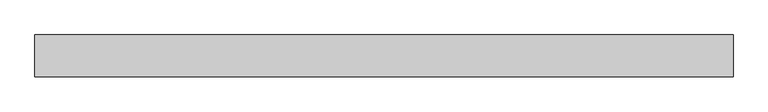
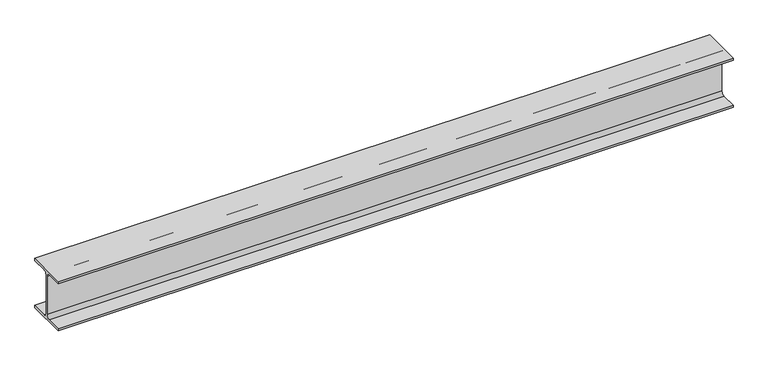
"""IFC4 building model written with IfcOpenShell, lengths in millimetres: beam geometry, 0912_Steel Framing_H-KSD3502 : H_SB_ASB_H-194x150x6x9."""

from ifc_helpers import new_model, si_unit, point, frame, frame_2d, origin, place, context, project, spatial, polyline, circle_curve, trimmed, segment, composite_curve, outline, extrude, source, transform, mapped, element, save


def beam_24c894de(model_context):
    return source(origin(), model_context, "Body", "SweptSolid", [
        extrude(outline(composite_curve([segment(polyline([(75.0, -88.0), (75.0, -97.0), (-75.0, -97.0), (-75.0, -88.0), (-16.0, -88.0)]), True, "CONTINUOUS"), segment(trimmed(circle_curve(frame_2d((-16.0, -75.0)), 13.0), [point((-16.0, -88.0))], [point((-3.0, -75.0))], True, "CARTESIAN"), True, "CONTINUOUS"), segment(polyline([(-3.0, -75.0), (-3.0, 75.0)]), True, "CONTINUOUS"), segment(trimmed(circle_curve(frame_2d((-16.0, 75.0)), 13.0), [point((-3.0, 75.0))], [point((-16.0, 88.0))], True, "CARTESIAN"), True, "CONTINUOUS"), segment(polyline([(-16.0, 88.0), (-75.0, 88.0), (-75.0, 97.0), (75.0, 97.0), (75.0, 88.0), (16.0, 88.0)]), True, "CONTINUOUS"), segment(trimmed(circle_curve(frame_2d((16.0, 75.0)), 13.0), [point((16.0, 88.0))], [point((3.0, 75.0))], True, "CARTESIAN"), True, "CONTINUOUS"), segment(polyline([(3.0, 75.0), (3.0, -75.0)]), True, "CONTINUOUS"), segment(trimmed(circle_curve(frame_2d((16.0, -75.0)), 13.0), [point((3.0, -75.0))], [point((16.0, -88.0))], True, "CARTESIAN"), True, "CONTINUOUS"), segment(polyline([(16.0, -88.0), (75.0, -88.0)]), True, "CONTINUOUS")], self_intersect=False)), frame((-1253.7727018, 0.0, 0.0), z_axis=(1.0, 0.0, 0.0), x_axis=(0.0, 1.0, 0.0)), (0.0, 0.0, 1.0), 2507.5454036),
    ])


if __name__ == "__main__":
    model = new_model("IFC4")
    model_context = context("Model", 3, world=origin())
    ifc_project = project(units=[si_unit("LENGTHUNIT", "METRE", prefix="MILLI")], contexts=[model_context])
    site = spatial("IfcSite", under=ifc_project)
    building = spatial("IfcBuilding", under=site)
    placement = place(None, origin())
    beam_shape = beam_24c894de(model_context)
    element("IfcBeam", 1, ObjectType="0912_Steel Framing_H-KSD3502 : H_SB_ASB_H-194x150x6x9", at=placement, inside=building, context=model_context, shape_type="MappedRepresentation", body=[
        mapped(beam_shape, transform((0.0, 0.0, 0.0), x_axis=(1.0, 0.0, 0.0), y_axis=(0.0, 1.0, 0.0), z_axis=(0.0, 0.0, 1.0))),
    ])
    save(model, "model.ifc")

# Revit data of these elements
# Type "0912_Steel Framing_H-KSD3502 : H_SB_ASB_H-194x150x6x9"
#   H_WM Code_1 = "S01AA002-00001 | Main Steel Structure Fabrication Work | Shelter/Building | Medium Steel - Standard (90KG/M>Weight≥30KG/M) | Material: (   )"
#   H_WM Code_2 = "S03AA028-00001 | Main Steel Structure Erection Work | Shelter/Building | Medium Steel (90KG/M>Weight≥30KG/M) | Material: (   )"
#   H_WM Code_3 = "S01AA010-00001 | Main Steel Structure Fabrication Work | Shelter/Building | Steel Painting/Coating | for Non-Fireproofed Steel Surface, Surface Preparation, Primer, Second & Final Coat | Material: (   )"
#   H_Q'ty Cal Type Tag = "SB-Q2"
#   Width = 15.0 cm
#   Web Thickness = 0.6 cm
#   Web Fillet = 1.3 cm
#   Warping Constant = 43316.0 cm⁶
#   W = 0
#   Torsional Moment of Inertia = 8.622 cm⁴
#   Section Area = 39.01 cm²
#   Plastic Modulus weak axis = 104.0 cm³
#   Plastic Modulus strong axis = 309.0 cm³
#   Perimeter = 0.95 m²/m
#   Nominal Weight = 30.60 kgf/m
#   Moment of Inertia weak axis = 507.00 cm⁴
#   Moment of Inertia strong axis = 2690.00 cm⁴
#   Height = 19.4 cm
#   Flange Thickness = 0.9 cm
#   Elastic Modulus weak axis = 67.6 cm³
#   Elastic Modulus strong axis = 277.0 cm³
#   Centroid Vertical = 9.7 cm
#   Centroid Horizontal = 7.5 cm
#   Ix = 26900000
#   Length [instance default] = 1.5240 m
#   Zx = 309000
#   b = 0.1500 m
#   h = 0.1940 m
#   r = 0.0130 m
#   s = 0.0060 m
#   t = 0.0090 m
#   A = 0.003901 m²
#   Structural Material [instance default] = Steel, 45-345
#   Assembly Code = ""
# Element 1 (IfcBeam, "0912_Steel Framing_H-KSD3502 : H_SB_ASB_H-194x150x6x9")
#   Structural Material = none
# Materials
#   "Steel, 45-345": class "Metal", colour RGB 189 187 185, transparency 0, Description = "Steel 345 MPa", Cost = 0
